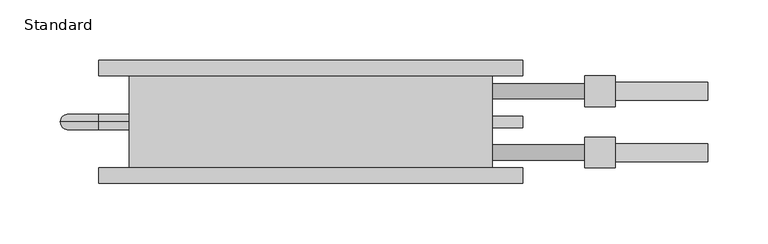
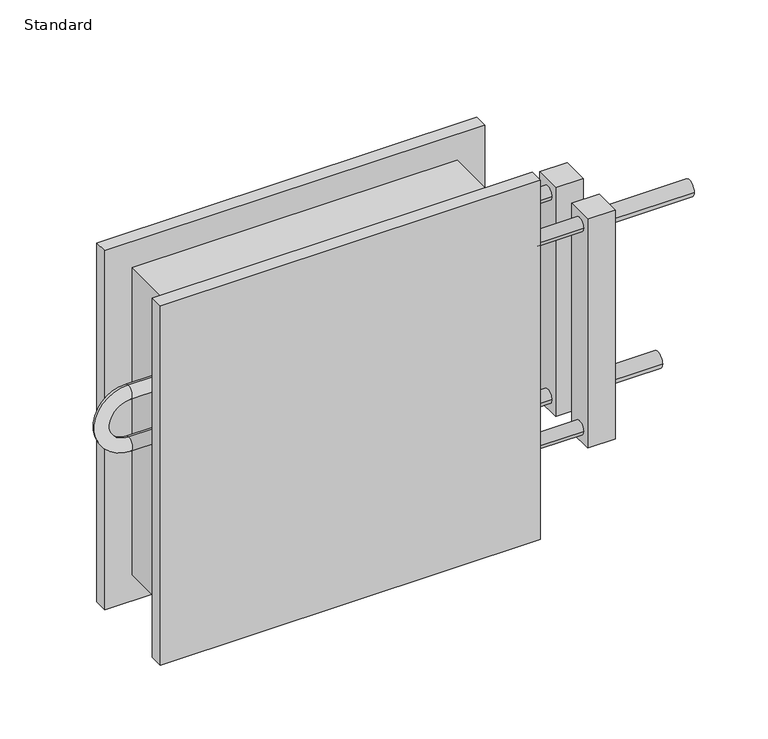
"""IFC4 building model written with IfcOpenShell, lengths in millimetres: proxy geometry, M_Coil - Chilled Water : Standard."""

from ifc_helpers import new_model, si_unit, point, frame, frame_2d, origin, place, context, project, spatial, circle_curve, ellipse_curve, trimmed, segment, composite_curve, outline, extrude, source, transform, mapped, element, save
from ifc_brep_helpers import plane_surface, cylinder_surface, revolved_surface, advanced_brep


def standard_6f93374b(model_context):
    return source(origin(), model_context, "Body", "SolidModel", [
        extrude(outline(composite_curve([segment(trimmed(circle_curve(frame_2d((38.1, 19.05)), 4.7625), [point((33.3375, 19.05))], [point((42.8625, 19.05))], False, "CARTESIAN"), True, "CONTINUOUS"), segment(trimmed(circle_curve(frame_2d((38.1, 19.05)), 4.7625), [point((42.8625, 19.05))], [point((33.3375, 19.05))], False, "CARTESIAN"), True, "CONTINUOUS")], self_intersect=False)), frame((150.0, 0.0, 0.0), z_axis=(1.0, 0.0, 0.0), x_axis=(0.0, 1.0, 0.0)), (0.0, 0.0, 1.0), 25.4),
        advanced_brep(
        [(-150.0, 76.2, 300.0), (-150.0, 0.0, 300.0), (150.0, 0.0, 300.0), (150.0, 76.2, 300.0), (150.0, 76.2, 0.0), (150.0, 0.0, 0.0), (-150.0, 0.0, 0.0), (-150.0, 76.2, 0.0), (-150.0, 38.1, 217.45), (-150.0, 38.1, 204.75), (-150.0, 38.1, 166.65), (-150.0, 38.1, 153.95), (150.0, 57.15, 249.2), (150.0, 69.85, 249.2), (150.0, 6.35, 50.8), (150.0, 19.05, 50.8), (150.0, 6.35, 249.2), (150.0, 19.05, 249.2), (150.0, 57.15, 50.8), (150.0, 69.85, 50.8), (175.4, 76.2, 325.4), (-175.4, 76.2, 325.4), (-175.4, 76.2, -25.4), (175.4, 76.2, -25.4), (175.4, 88.9, 325.4), (175.4, 88.9, -25.4), (-175.4, 88.9, -25.4), (-175.4, 88.9, 325.4), (328.05, 56.0, 50.8), (328.05, 71.0, 50.8), (328.05, 5.2, 249.2), (328.05, 20.2, 249.2), (251.85, 56.0, 50.8), (251.85, 71.0, 50.8), (251.85, 5.2, 249.2), (251.85, 20.2, 249.2), (175.4, -12.7, 325.4), (-175.4, -12.7, 325.4), (-175.4, -12.7, -25.4), (175.4, -12.7, -25.4), (175.4, 0.0, 325.4), (175.4, 0.0, -25.4), (-175.4, 0.0, -25.4), (-175.4, 0.0, 325.4), (-175.4, 38.1, 217.45), (-175.4, 38.1, 204.75), (-175.4, 38.1, 153.95), (-175.4, 38.1, 166.65), (226.45, 57.15, 249.2), (226.45, 69.85, 249.2), (226.45, 6.35, 50.8), (226.45, 19.05, 50.8), (226.45, 6.35, 249.2), (226.45, 19.05, 249.2), (226.45, 57.15, 50.8), (226.45, 69.85, 50.8), (251.85, 50.8, 261.9), (251.85, 50.8, 38.1), (251.85, 76.2, 38.1), (251.85, 76.2, 261.9), (251.85, 0.0, 261.9), (251.85, 0.0, 38.1), (251.85, 25.4, 38.1), (251.85, 25.4, 261.9), (226.45, 50.8, 261.9), (226.45, 76.2, 261.9), (226.45, 76.2, 38.1), (226.45, 50.8, 38.1), (226.45, 0.0, 261.9), (226.45, 25.4, 261.9), (226.45, 25.4, 38.1), (226.45, 0.0, 38.1)],
        [
            (0, 1),
            (1, 2),
            (2, 3),
            (3, 0),
            (4, 5),
            (5, 6),
            (6, 7),
            (7, 4),
            (0, 7),
            (6, 1),
            (8, 9, circle_curve(frame((-150.0, 38.1, 211.1), z_axis=(1.0, 0.0, 0.0), x_axis=(0.0, 0.0, -1.0)), 6.35)),
            (9, 8, circle_curve(frame((-150.0, 38.1, 211.1), z_axis=(1.0, 0.0, 0.0), x_axis=(0.0, 0.0, -1.0)), 6.35)),
            (10, 11, circle_curve(frame((-150.0, 38.1, 160.3), z_axis=(1.0, 0.0, 0.0), x_axis=(0.0, 0.0, 1.0)), 6.35)),
            (11, 10, circle_curve(frame((-150.0, 38.1, 160.3), z_axis=(1.0, 0.0, 0.0), x_axis=(0.0, 0.0, 1.0)), 6.35)),
            (2, 5),
            (4, 3),
            (12, 13, circle_curve(frame((150.0, 63.5, 249.2), z_axis=(-1.0, 0.0, 0.0), x_axis=(0.0, 1.0, 0.0)), 6.35)),
            (13, 12, circle_curve(frame((150.0, 63.5, 249.2), z_axis=(-1.0, 0.0, 0.0), x_axis=(0.0, 1.0, 0.0)), 6.35)),
            (14, 15, circle_curve(frame((150.0, 12.7, 50.8), z_axis=(-1.0, 0.0, 0.0), x_axis=(0.0, 1.0, 0.0)), 6.35)),
            (15, 14, circle_curve(frame((150.0, 12.7, 50.8), z_axis=(-1.0, 0.0, 0.0), x_axis=(0.0, 1.0, 0.0)), 6.35)),
            (16, 17, circle_curve(frame((150.0, 12.7, 249.2), z_axis=(-1.0, 0.0, 0.0), x_axis=(0.0, 1.0, 0.0)), 6.35)),
            (17, 16, circle_curve(frame((150.0, 12.7, 249.2), z_axis=(-1.0, 0.0, 0.0), x_axis=(0.0, 1.0, 0.0)), 6.35)),
            (18, 19, circle_curve(frame((150.0, 63.5, 50.8), z_axis=(-1.0, 0.0, 0.0), x_axis=(0.0, 1.0, 0.0)), 6.35)),
            (19, 18, circle_curve(frame((150.0, 63.5, 50.8), z_axis=(-1.0, 0.0, 0.0), x_axis=(0.0, 1.0, 0.0)), 6.35)),
            (20, 21),
            (21, 22),
            (22, 23),
            (23, 20),
            (24, 25),
            (25, 26),
            (26, 27),
            (27, 24),
            (20, 24),
            (27, 21),
            (26, 22),
            (25, 23),
            (28, 29, circle_curve(frame((328.05, 63.5, 50.8), z_axis=(1.0, 0.0, 0.0), x_axis=(0.0, 1.0, 0.0)), 7.5)),
            (29, 28, circle_curve(frame((328.05, 63.5, 50.8), z_axis=(1.0, 0.0, 0.0), x_axis=(0.0, 1.0, 0.0)), 7.5)),
            (30, 31, circle_curve(frame((328.05, 12.7, 249.2), z_axis=(1.0, 0.0, 0.0), x_axis=(0.0, 1.0, 0.0)), 7.5)),
            (31, 30, circle_curve(frame((328.05, 12.7, 249.2), z_axis=(1.0, 0.0, 0.0), x_axis=(0.0, 1.0, 0.0)), 7.5)),
            (28, 32),
            (32, 33, circle_curve(frame((251.85, 63.5, 50.8), z_axis=(1.0, 0.0, 0.0), x_axis=(0.0, 1.0, 0.0)), 7.5)),
            (33, 29),
            (33, 32, circle_curve(frame((251.85, 63.5, 50.8), z_axis=(1.0, 0.0, 0.0), x_axis=(0.0, 1.0, 0.0)), 7.5)),
            (30, 34),
            (34, 35, circle_curve(frame((251.85, 12.7, 249.2), z_axis=(1.0, 0.0, 0.0), x_axis=(0.0, 1.0, 0.0)), 7.5)),
            (35, 31),
            (35, 34, circle_curve(frame((251.85, 12.7, 249.2), z_axis=(1.0, 0.0, 0.0), x_axis=(0.0, 1.0, 0.0)), 7.5)),
            (36, 37),
            (37, 38),
            (38, 39),
            (39, 36),
            (40, 41),
            (41, 42),
            (42, 43),
            (43, 40),
            (36, 40),
            (43, 37),
            (42, 38),
            (41, 39),
            (8, 44),
            (44, 45, circle_curve(frame((-175.4, 38.1, 211.1), z_axis=(1.0, 0.0, 0.0), x_axis=(0.0, 0.0, -1.0)), 6.35)),
            (45, 9),
            (45, 44, circle_curve(frame((-175.4, 38.1, 211.1), z_axis=(1.0, 0.0, 0.0), x_axis=(0.0, 0.0, -1.0)), 6.35)),
            (44, 46, circle_curve(frame((-175.4, 38.1, 185.7), z_axis=(0.0, -1.0, 0.0), x_axis=(0.0, 0.0, 1.0)), 31.75)),
            (46, 47, circle_curve(frame((-175.4, 38.1, 160.3), z_axis=(-1.0, 0.0, 0.0), x_axis=(0.0, 0.0, 1.0)), 6.35)),
            (47, 45, circle_curve(frame((-175.4, 38.1, 185.7), z_axis=(0.0, 1.0, 0.0), x_axis=(0.0, 0.0, 1.0)), 19.05)),
            (47, 46, circle_curve(frame((-175.4, 38.1, 160.3), z_axis=(-1.0, 0.0, 0.0), x_axis=(0.0, 0.0, 1.0)), 6.35)),
            (46, 11),
            (10, 47),
            (12, 48),
            (48, 49, circle_curve(frame((226.45, 63.5, 249.2), z_axis=(-1.0, 0.0, 0.0), x_axis=(0.0, 1.0, 0.0)), 6.35)),
            (49, 13),
            (49, 48, circle_curve(frame((226.45, 63.5, 249.2), z_axis=(-1.0, 0.0, 0.0), x_axis=(0.0, 1.0, 0.0)), 6.35)),
            (14, 50),
            (50, 51, circle_curve(frame((226.45, 12.7, 50.8), z_axis=(-1.0, 0.0, 0.0), x_axis=(0.0, 1.0, 0.0)), 6.35)),
            (51, 15),
            (51, 50, circle_curve(frame((226.45, 12.7, 50.8), z_axis=(-1.0, 0.0, 0.0), x_axis=(0.0, 1.0, 0.0)), 6.35)),
            (16, 52),
            (52, 53, circle_curve(frame((226.45, 12.7, 249.2), z_axis=(-1.0, 0.0, 0.0), x_axis=(0.0, 1.0, 0.0)), 6.35)),
            (53, 17),
            (53, 52, circle_curve(frame((226.45, 12.7, 249.2), z_axis=(-1.0, 0.0, 0.0), x_axis=(0.0, 1.0, 0.0)), 6.35)),
            (18, 54),
            (54, 55, circle_curve(frame((226.45, 63.5, 50.8), z_axis=(-1.0, 0.0, 0.0), x_axis=(0.0, 1.0, 0.0)), 6.35)),
            (55, 19),
            (55, 54, circle_curve(frame((226.45, 63.5, 50.8), z_axis=(-1.0, 0.0, 0.0), x_axis=(0.0, 1.0, 0.0)), 6.35)),
            (56, 57),
            (57, 58),
            (58, 59),
            (59, 56),
            (60, 61),
            (61, 62),
            (62, 63),
            (63, 60),
            (64, 65),
            (65, 66),
            (66, 67),
            (67, 64),
            (68, 69),
            (69, 70),
            (70, 71),
            (71, 68),
            (56, 64),
            (67, 57),
            (66, 58),
            (65, 59),
            (60, 68),
            (71, 61),
            (70, 62),
            (69, 63),
        ],
        [
            plane_surface(frame((-150.0, 76.2, 300.0), z_axis=(0.0, 0.0, 1.0), x_axis=(-1.0, 0.0, 0.0))),
            plane_surface(frame((-150.0, 76.2, 0.0), z_axis=(0.0, 0.0, -1.0), x_axis=(1.0, 0.0, 0.0))),
            plane_surface(frame((-150.0, 76.2, 300.0), z_axis=(-1.0, 0.0, 0.0), x_axis=(0.0, 0.0, -1.0))),
            plane_surface(frame((150.0, 0.0, 300.0), z_axis=(1.0, 0.0, 0.0), x_axis=(0.0, 0.0, -1.0))),
            plane_surface(frame((-175.4, 76.2, 325.4), z_axis=(0.0, -1.0, 0.0), x_axis=(-1.0, 0.0, 0.0))),
            plane_surface(frame((-175.4, 88.9, 325.4), z_axis=(0.0, 1.0, 0.0), x_axis=(1.0, 0.0, 0.0))),
            plane_surface(frame((175.4, 76.2, 325.4), z_axis=(0.0, 0.0, 1.0), x_axis=(0.0, 1.0, 0.0))),
            plane_surface(frame((-175.4, 76.2, 325.4), z_axis=(-1.0, 0.0, 0.0), x_axis=(0.0, 1.0, 0.0))),
            plane_surface(frame((-175.4, 76.2, -25.4), z_axis=(0.0, 0.0, -1.0), x_axis=(0.0, 1.0, 0.0))),
            plane_surface(frame((175.4, 76.2, -25.4), z_axis=(1.0, 0.0, 0.0), x_axis=(0.0, 1.0, 0.0))),
            plane_surface(frame((328.05, 71.0, 50.8), z_axis=(1.0, 0.0, 0.0), x_axis=(0.0, 0.0, 1.0))),
            cylinder_surface(frame((251.85, 63.5, 50.8), z_axis=(1.0, 0.0, 0.0), x_axis=(0.0, 1.0, 0.0)), 7.5),
            cylinder_surface(frame((0.0, 12.7, 249.2), z_axis=(1.0, 0.0, 0.0), x_axis=(0.0, 1.0, 0.0)), 7.5),
            plane_surface(frame((-175.4, -12.7, 325.4), z_axis=(0.0, -1.0, 0.0), x_axis=(-1.0, 0.0, 0.0))),
            plane_surface(frame((-175.4, 0.0, 325.4), z_axis=(0.0, 1.0, 0.0), x_axis=(1.0, 0.0, 0.0))),
            plane_surface(frame((175.4, -12.7, 325.4), z_axis=(0.0, 0.0, 1.0), x_axis=(0.0, 1.0, 0.0))),
            plane_surface(frame((-175.4, -12.7, 325.4), z_axis=(-1.0, 0.0, 0.0), x_axis=(0.0, 1.0, 0.0))),
            plane_surface(frame((-175.4, -12.7, -25.4), z_axis=(0.0, 0.0, -1.0), x_axis=(0.0, 1.0, 0.0))),
            plane_surface(frame((175.4, -12.7, -25.4), z_axis=(1.0, 0.0, 0.0), x_axis=(0.0, 1.0, 0.0))),
            cylinder_surface(frame((-150.0, 38.1, 211.1), z_axis=(1.0, 0.0, 0.0), x_axis=(0.0, 0.0, -1.0)), 6.35),
            revolved_surface(trimmed(ellipse_curve(frame((-175.4, 38.1, 211.1), z_axis=(1.0, 0.0, 0.0), x_axis=(0.0, 0.0, -1.0)), 6.35, 6.35), [point((-175.4, 38.1, 217.45))], [point((-175.4, 38.1, 204.75))], True, "CARTESIAN"), (-175.4, 0.0, 185.7), (0.0, -1.0, 0.0)),
            revolved_surface(trimmed(ellipse_curve(frame((-175.4, 38.1, 211.1), z_axis=(1.0, 0.0, 0.0), x_axis=(0.0, 0.0, -1.0)), 6.35, 6.35), [point((-175.4, 38.1, 204.75))], [point((-175.4, 38.1, 217.45))], True, "CARTESIAN"), (-175.4, 0.0, 185.7), (0.0, -1.0, 0.0)),
            cylinder_surface(frame((-175.4, 38.1, 160.3), z_axis=(-1.0, 0.0, 0.0), x_axis=(0.0, 0.0, 1.0)), 6.35),
            cylinder_surface(frame((150.0, 63.5, 249.2), z_axis=(-1.0, 0.0, 0.0), x_axis=(0.0, 1.0, 0.0)), 6.35),
            cylinder_surface(frame((150.0, 12.7, 50.8), z_axis=(-1.0, 0.0, 0.0), x_axis=(0.0, 1.0, 0.0)), 6.35),
            cylinder_surface(frame((150.0, 12.7, 249.2), z_axis=(-1.0, 0.0, 0.0), x_axis=(0.0, 1.0, 0.0)), 6.35),
            cylinder_surface(frame((150.0, 63.5, 50.8), z_axis=(-1.0, 0.0, 0.0), x_axis=(0.0, 1.0, 0.0)), 6.35),
            plane_surface(frame((251.85, 50.8, 261.9), z_axis=(1.0, 0.0, 0.0), x_axis=(0.0, 0.0, -1.0))),
            plane_surface(frame((226.45, 50.8, 261.9), z_axis=(-1.0, 0.0, 0.0), x_axis=(0.0, 0.0, 1.0))),
            plane_surface(frame((251.85, 50.8, 261.9), z_axis=(0.0, -1.0, 0.0), x_axis=(-1.0, 0.0, 0.0))),
            plane_surface(frame((251.85, 50.8, 38.1), z_axis=(0.0, 0.0, -1.0), x_axis=(-1.0, 0.0, 0.0))),
            plane_surface(frame((251.85, 76.2, 38.1), z_axis=(0.0, 1.0, 0.0), x_axis=(-1.0, 0.0, 0.0))),
            plane_surface(frame((251.85, 76.2, 261.9), z_axis=(0.0, 0.0, 1.0), x_axis=(-1.0, 0.0, 0.0))),
            plane_surface(frame((251.85, 0.0, 261.9), z_axis=(0.0, -1.0, 0.0), x_axis=(-1.0, 0.0, 0.0))),
            plane_surface(frame((251.85, 0.0, 38.1), z_axis=(0.0, 0.0, -1.0), x_axis=(-1.0, 0.0, 0.0))),
            plane_surface(frame((251.85, 25.4, 38.1), z_axis=(0.0, 1.0, 0.0), x_axis=(-1.0, 0.0, 0.0))),
            plane_surface(frame((251.85, 25.4, 261.9), z_axis=(0.0, 0.0, 1.0), x_axis=(-1.0, 0.0, 0.0))),
        ],
        [
            (0, [[1, 2, 3, 4]]),
            (1, [[5, 6, 7, 8]]),
            (2, [[-1, 9, -7, 10], [11, 12], [13, 14]]),
            (3, [[-3, 15, -5, 16], [17, 18], [19, 20], [21, 22], [23, 24]]),
            (4, [[25, 26, 27, 28], [-4, -16, -8, -9]]),
            (5, [[29, 30, 31, 32]]),
            (6, [[-25, 33, -32, 34]]),
            (7, [[-26, -34, -31, 35]]),
            (8, [[-27, -35, -30, 36]]),
            (9, [[-28, -36, -29, -33]]),
            (10, [[37, 38]]),
            (10, [[39, 40]]),
            (11, [[-37, 41, 42, 43]]),
            (11, [[-38, -43, 44, -41]]),
            (12, [[-39, 45, 46, 47]]),
            (12, [[-40, -47, 48, -45]]),
            (13, [[49, 50, 51, 52]]),
            (14, [[53, 54, 55, 56], [-2, -10, -6, -15]]),
            (15, [[-49, 57, -56, 58]]),
            (16, [[-50, -58, -55, 59]]),
            (17, [[-51, -59, -54, 60]]),
            (18, [[-52, -60, -53, -57]]),
            (19, [[61, 62, 63, -11]]),
            (19, [[-61, -12, -63, 64]]),
            (20, [[-62, 65, 66, 67]]),
            (21, [[-64, -67, 68, -65]]),
            (22, [[-66, 69, -13, 70]]),
            (22, [[-68, -70, -14, -69]]),
            (23, [[71, 72, 73, -17]]),
            (23, [[-71, -18, -73, 74]]),
            (24, [[75, 76, 77, -19]]),
            (24, [[-75, -20, -77, 78]]),
            (25, [[79, 80, 81, -21]]),
            (25, [[-79, -22, -81, 82]]),
            (26, [[83, 84, 85, -23]]),
            (26, [[-83, -24, -85, 86]]),
            (27, [[87, 88, 89, 90], [-42, -44]]),
            (27, [[91, 92, 93, 94], [-46, -48]]),
            (28, [[95, 96, 97, 98], [-72, -74], [-84, -86]]),
            (28, [[99, 100, 101, 102], [-76, -78], [-80, -82]]),
            (29, [[-87, 103, -98, 104]]),
            (30, [[-88, -104, -97, 105]]),
            (31, [[-89, -105, -96, 106]]),
            (32, [[-90, -106, -95, -103]]),
            (33, [[-91, 107, -102, 108]]),
            (34, [[-92, -108, -101, 109]]),
            (35, [[-93, -109, -100, 110]]),
            (36, [[-94, -110, -99, -107]]),
        ],
    ),
    ])


if __name__ == "__main__":
    model = new_model("IFC4")
    model_context = context("Model", 3, world=origin())
    ifc_project = project(units=[si_unit("LENGTHUNIT", "METRE", prefix="MILLI")], contexts=[model_context])
    site = spatial("IfcSite", under=ifc_project)
    building = spatial("IfcBuilding", under=site)
    placement = place(None, origin())
    standard_shape = standard_6f93374b(model_context)
    element("IfcBuildingElementProxy", 1, Name="M_Coil - Chilled Water : Standard", ObjectType="M_Coil - Chilled Water : Standard", at=placement, inside=building, context=model_context, shape_type="MappedRepresentation", body=[
        mapped(standard_shape, transform((0.0, 0.0, 0.0), x_axis=(1.0, 0.0, 0.0), y_axis=(0.0, 1.0, 0.0), z_axis=(0.0, 0.0, 1.0))),
    ])
    save(model, "model.ifc")

# Revit data of these elements
# Project information
#   Project Issue Date = "Issue Date"
#   Project Status = "Project Status"
#   Client Name = "Owner"
#   Project Address = "Enter address here"
#   Project Name = "Project Name"
#   Project Number = "Project Number"
# Type "M_Coil - Chilled Water : Standard"
#   Duct Width [instance default] = 300 mm
#   Duct Height [instance default] = 300 mm
#   Drain Flow [instance default] = 0.0 L/s
#   Coil Length [instance default] = 459 mm
#   Water Radius = 7.5 mm
#   Water Pressure Drop [instance default] = 0 kPa
#   Water Flow [instance default] = 0.0 L/s
#   Water Diameter = 15 mm
#   Air Pressure Drop [instance default] = 8.0 Pa
#   Air Flow [instance default] = 236.0 L/s
#   Coil Material = none
# Element 1 (IfcBuildingElementProxy, "M_Coil - Chilled Water : Standard")
#   Water Pressure Drop = 140 kPa
#   Water Flow = 10.0 L/s
